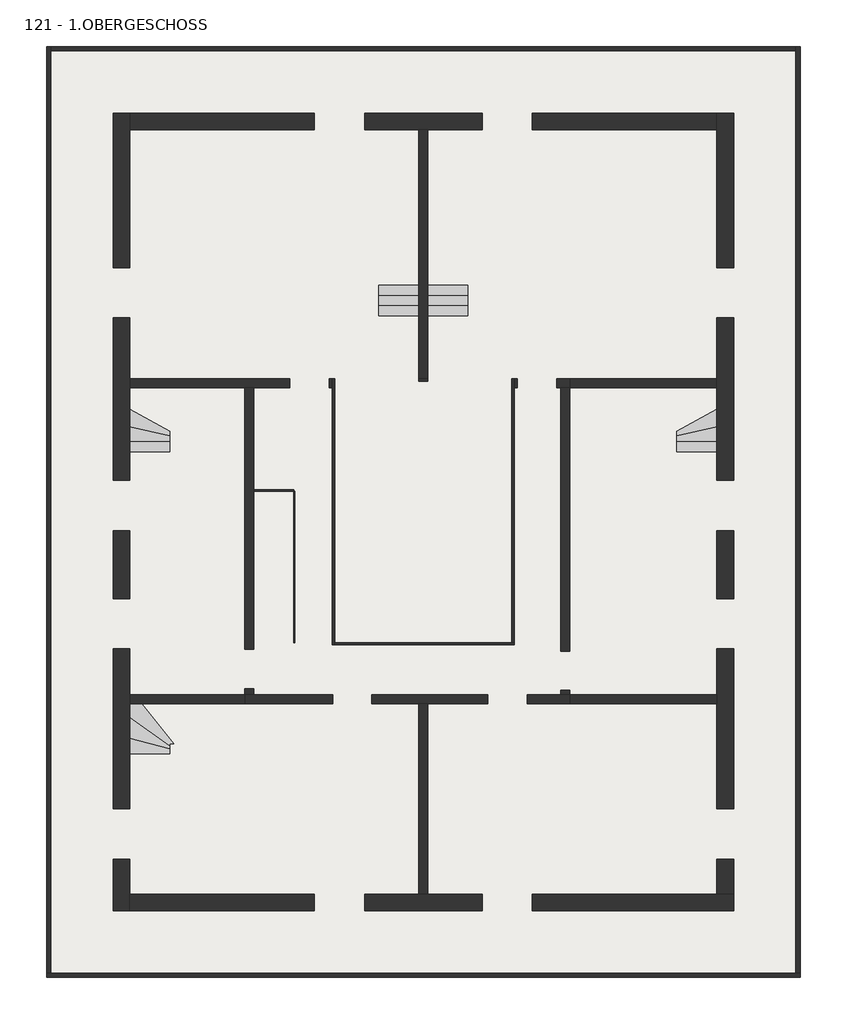
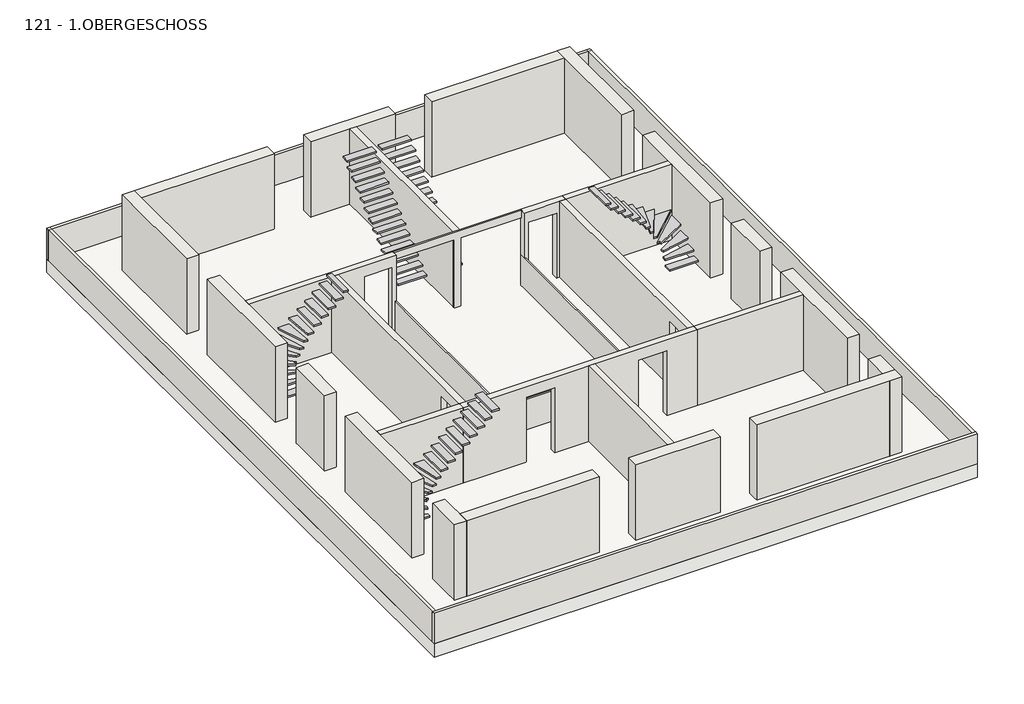
# One storey: 24 walls, 10 stairs, 1 slab.
"""IFC4 building model written with IfcOpenShell, lengths in millimetres."""

import ifcopenshell
import ifcopenshell.guid

model = None  # the IFC model being written
_history = None  # IfcOwnerHistory: only IFC2X3 demands one
_inside = {}  # id of a spatial element -> (the spatial element, [elements in it])
_under = {}  # id of a project, library or spatial element -> (it, [spatial elements below it])
_declared = {}  # id of a project -> (the project, [libraries it declares])
_typed = {}  # id of a type object -> (the type object, [elements of that type])
_made_of = {}  # id of a material, layer set ... -> (it, [elements and type objects made of it])


def new_model(schema):
    """Start an empty IFC model of exactly this schema.

    Asked for "IFC4X3", IfcOpenShell would pick the latest addendum, in which some entities
    have other attributes; the version numbers below select the first issue.
    IFC2X3 requires an IfcOwnerHistory on every rooted entity: one is made here for all.
    """
    global model, _history
    if schema == "IFC4X3":
        model = ifcopenshell.file(schema_version=(4, 3, 0, 0))
    else:
        model = ifcopenshell.file(schema=schema)
    _inside.clear()
    _under.clear()
    _declared.clear()
    _typed.clear()
    _made_of.clear()
    _history = None
    if model.schema == "IFC2X3":
        org = make("IfcOrganization", Name="unknown")
        user = make(
            "IfcPersonAndOrganization",
            ThePerson=make("IfcPerson", FamilyName="unknown"),
            TheOrganization=org,
        )
        app = make(
            "IfcApplication",
            ApplicationDeveloper=org,
            Version="unknown",
            ApplicationFullName="unknown",
            ApplicationIdentifier="unknown",
        )
        _history = make(
            "IfcOwnerHistory",
            OwningUser=user,
            OwningApplication=app,
            ChangeAction="ADDED",
            CreationDate=0,
        )
    return model


def make(cls, **values):
    """One entity of the class cls with the attributes given. An attribute that is None is left unset."""
    return model.create_entity(
        cls, **{name: value for name, value in values.items() if value is not None}
    )


def rooted(cls, **values):
    """An entity with a GlobalId (a new one), such as an element, a storey or a relation."""
    return make(cls, GlobalId=ifcopenshell.guid.new(), OwnerHistory=_history, **values)


def si_unit(unit_type, name, prefix=None):
    """IfcSIUnit, for example si_unit("LENGTHUNIT", "METRE", prefix="MILLI")."""
    return make("IfcSIUnit", UnitType=unit_type, Prefix=prefix, Name=name)


def assignment(units):
    """IfcUnitAssignment: the units of a project."""
    return None if units is None else make("IfcUnitAssignment", Units=units)


def point(xyz):
    """IfcCartesianPoint."""
    return None if xyz is None else make("IfcCartesianPoint", Coordinates=xyz)


def direction(xyz):
    """IfcDirection."""
    return None if xyz is None else make("IfcDirection", DirectionRatios=xyz)


def frame(location, z_axis=None, x_axis=None):
    """IfcAxis2Placement3D, a coordinate frame: its origin and axes. An axis left out is left unset."""
    return make(
        "IfcAxis2Placement3D",
        Location=point(location),
        Axis=direction(z_axis),
        RefDirection=direction(x_axis),
    )


def origin():
    """The frame at (0, 0, 0) with its axes left unset."""
    return frame((0.0, 0.0, 0.0))


def place(relative_to, where):
    """IfcLocalPlacement: puts the frame where relative to a parent placement (None: the world)."""
    return make(
        "IfcLocalPlacement", PlacementRelTo=relative_to, RelativePlacement=where
    )


def context(
    kind, dimensions, precision=None, world=None, true_north=None, identifier=None
):
    """IfcGeometricRepresentationContext, for example the 3D "Model" context."""
    return make(
        "IfcGeometricRepresentationContext",
        ContextIdentifier=identifier,
        ContextType=kind,
        CoordinateSpaceDimension=dimensions,
        Precision=precision,
        WorldCoordinateSystem=world,
        TrueNorth=true_north,
    )


def project(units=None, contexts=None):
    """IfcProject with its units and contexts."""
    return rooted(
        "IfcProject",
        Name="project",
        RepresentationContexts=contexts,
        UnitsInContext=assignment(units),
    )


def spatial(cls, under=None, at=None, **own):
    """A site, building, storey or space (cls), placed at a placement, below another one or the project."""
    s = rooted(cls, ObjectPlacement=at, **own)
    if under is not None:
        _under.setdefault(under.id(), (under, []))[1].append(s)
    return s


def polyline(points):
    """IfcPolyline through the points."""
    return make("IfcPolyline", Points=[point(p) for p in points])


def outline(outer, holes=None, kind="AREA"):
    """IfcArbitraryClosedProfileDef: a profile drawn as a closed curve; with holes, ...WithVoids."""
    if holes is None:
        return make("IfcArbitraryClosedProfileDef", ProfileType=kind, OuterCurve=outer)
    return make(
        "IfcArbitraryProfileDefWithVoids",
        ProfileType=kind,
        OuterCurve=outer,
        InnerCurves=holes,
    )


def extrude(swept, where, along, depth):
    """IfcExtrudedAreaSolid: the profile swept, set in the frame where, extruded along a direction by depth."""
    return make(
        "IfcExtrudedAreaSolid",
        SweptArea=swept,
        Position=where,
        ExtrudedDirection=direction(along),
        Depth=depth,
    )


def shape(context_of_items, identifier, shape_type, items):
    """IfcShapeRepresentation: the items that make up one representation, for example the "Body"."""
    return make(
        "IfcShapeRepresentation",
        ContextOfItems=context_of_items,
        RepresentationIdentifier=identifier,
        RepresentationType=shape_type,
        Items=items,
    )


def source(mapping_origin, context_of_items, identifier, shape_type, items):
    """IfcRepresentationMap: a shape defined once, which mapped items show again and again."""
    return make(
        "IfcRepresentationMap",
        MappingOrigin=mapping_origin,
        MappedRepresentation=shape(context_of_items, identifier, shape_type, items),
    )


def transform(
    local_origin,
    x_axis=None,
    y_axis=None,
    z_axis=None,
    scale=None,
    scale2=None,
    scale3=None,
    uniform=True,
):
    """IfcCartesianTransformationOperator3D, or its non-uniform kind. x_axis, y_axis, z_axis: its Axis1, 2, 3."""
    if uniform:
        return make(
            "IfcCartesianTransformationOperator3D",
            Axis1=direction(x_axis),
            Axis2=direction(y_axis),
            LocalOrigin=point(local_origin),
            Scale=scale,
            Axis3=direction(z_axis),
        )
    return make(
        "IfcCartesianTransformationOperator3DnonUniform",
        Axis1=direction(x_axis),
        Axis2=direction(y_axis),
        LocalOrigin=point(local_origin),
        Scale=scale,
        Axis3=direction(z_axis),
        Scale2=scale2,
        Scale3=scale3,
    )


def mapped(mapping_source, mapping_target):
    """IfcMappedItem: shows the shape of a source again, moved by a transform."""
    return make(
        "IfcMappedItem", MappingSource=mapping_source, MappingTarget=mapping_target
    )


def made_of(thing, what):
    """Note that an element or type object is made of a material, layer set ...; save() writes the relation."""
    if what is not None:
        _made_of.setdefault(what.id(), (what, []))[1].append(thing)
    return thing


def element(
    cls,
    number,
    at=None,
    inside=None,
    cuts=None,
    type_object=None,
    material=None,
    context=None,
    identifier="Body",
    shape_type=None,
    held_by="IfcProductDefinitionShape",
    body=None,
    shapes=None,
    **own,
):
    """One element of the class cls, such as IfcWall. Its Tag is "e" and its number.

    at: its placement. inside: the storey or other place that contains it. cuts: it is an
    opening in that element (IfcRelVoidsElement). A single representation is given by context,
    identifier, shape_type and body (its items); several are given by shapes. held_by: the class
    of the entity that holds the representations. save() writes the other relations.
    """
    e = rooted(cls, Tag="e%d" % number, ObjectPlacement=at, **own)
    if body is not None:
        shapes = [shape(context, identifier, shape_type, body)]
    if shapes is not None:
        e.Representation = make(held_by, Representations=shapes)
    if inside is not None:
        _inside.setdefault(inside.id(), (inside, []))[1].append(e)
    if cuts is not None:
        rooted(
            "IfcRelVoidsElement", RelatingBuildingElement=cuts, RelatedOpeningElement=e
        )
    if type_object is not None:
        _typed.setdefault(type_object.id(), (type_object, []))[1].append(e)
    return made_of(e, material)


def aggregate(whole, parts):
    """IfcRelAggregates: a whole, such as a stair, and the parts it consists of."""
    return rooted("IfcRelAggregates", RelatingObject=whole, RelatedObjects=parts)


def save(model, path):
    """Write the relations noted so far, then the file.

    IfcRelAggregates (storeys below a building ...), IfcRelContainedInSpatialStructure (elements
    in a storey), IfcRelDefinesByType, IfcRelAssociatesMaterial and IfcRelDeclares: one each for
    every whole, place, type object, material and project.
    """
    for whole, parts in _under.values():
        aggregate(whole, parts)
    for where, things in _inside.values():
        rooted(
            "IfcRelContainedInSpatialStructure",
            RelatedElements=things,
            RelatingStructure=where,
        )
    for kind, things in _typed.values():
        rooted("IfcRelDefinesByType", RelatedObjects=things, RelatingType=kind)
    for what, things in _made_of.values():
        rooted("IfcRelAssociatesMaterial", RelatedObjects=things, RelatingMaterial=what)
    for by, libraries in _declared.values():
        rooted("IfcRelDeclares", RelatingContext=by, RelatedDefinitions=libraries)
    model.write(path)


def slab_4f2d1623(model_context):
    return source(origin(), model_context, "Body", "SweptSolid", [
        extrude(outline(polyline([(174297.7593015, 47984.7962965), (174297.7593015, 26981.9343946), (157297.7593015, 26981.9343946), (157297.7593015, 47984.7962965), (174297.7593015, 47984.7962965)])), frame((0.0, 0.0, 2880.0), z_axis=(0.0, 0.0, 1.0), x_axis=(1.0, 0.0, 0.0)), (0.0, 0.0, 1.0), 450.0),
    ])


def stair_92ba3d55(model_context):
    return source(origin(), model_context, "Body", "SweptSolid", [
        extrude(outline(polyline([(160077.7593015, 32139.1812131), (160077.7593015, 32029.7962965), (159177.7593015, 32029.7962965), (159177.7593015, 32381.5903923), (160077.7593015, 32139.1812131)])), frame((0.0, 0.0, 3480.0), z_axis=(0.0, 0.0, 1.0), x_axis=(1.0, 0.0, 0.0)), (0.0, 0.0, 1.0), 50.0),
        extrude(outline(polyline([(160077.7593015, 32208.6851854), (160077.7593015, 32139.1812131), (159177.7593015, 32381.5903923), (159177.7593015, 32851.1265298), (160077.7593015, 32208.6851854)])), frame((0.0, 0.0, 3680.0), z_axis=(0.0, 0.0, 1.0), x_axis=(1.0, 0.0, 0.0)), (0.0, 0.0, 1.0), 50.0),
        extrude(outline(polyline([(159450.38828, 33159.7962965), (160164.4298971, 32259.7962965), (160077.7593015, 32259.7962965), (160077.7593015, 32208.6851854), (159177.7593015, 32851.1265298), (159177.7593015, 33159.7962965), (159450.38828, 33159.7962965)])), frame((0.0, 0.0, 3880.0), z_axis=(0.0, 0.0, 1.0), x_axis=(1.0, 0.0, 0.0)), (0.0, 0.0, 1.0), 50.0),
        extrude(outline(polyline([(160285.4396784, 32259.7962965), (160164.4298971, 32259.7962965), (159450.38828, 33159.7962965), (159877.5404106, 33159.7962965), (160285.4396784, 32259.7962965)])), frame((0.0, 0.0, 4080.0), z_axis=(0.0, 0.0, 1.0), x_axis=(1.0, 0.0, 0.0)), (0.0, 0.0, 1.0), 50.0),
        extrude(outline(polyline([(160412.2916695, 32259.7962965), (160285.4396784, 32259.7962965), (159877.5404106, 33159.7962965), (160212.4306066, 33159.7962965), (160412.2916695, 32259.7962965)])), frame((0.0, 0.0, 4280.0), z_axis=(0.0, 0.0, 1.0), x_axis=(1.0, 0.0, 0.0)), (0.0, 0.0, 1.0), 50.0),
        extrude(outline(polyline([(160546.5910216, 32259.7962965), (160412.2916695, 32259.7962965), (160212.4306066, 33159.7962965), (160538.1312545, 33159.7962965), (160546.5910216, 32259.7962965)])), frame((0.0, 0.0, 4480.0), z_axis=(0.0, 0.0, 1.0), x_axis=(1.0, 0.0, 0.0)), (0.0, 0.0, 1.0), 50.0),
        extrude(outline(polyline([(160772.3611381, 32259.7962965), (160546.5910216, 32259.7962965), (160538.1312545, 33159.7962965), (160772.3611381, 33159.7962965), (160772.3611381, 32259.7962965)])), frame((0.0, 0.0, 4680.0), z_axis=(0.0, 0.0, 1.0), x_axis=(1.0, 0.0, 0.0)), (0.0, 0.0, 1.0), 50.0),
        extrude(outline(polyline([(161002.3611381, 32259.7962965), (160772.3611381, 32259.7962965), (160772.3611381, 33159.7962965), (161002.3611381, 33159.7962965), (161002.3611381, 32259.7962965)])), frame((0.0, 0.0, 4880.0), z_axis=(0.0, 0.0, 1.0), x_axis=(1.0, 0.0, 0.0)), (0.0, 0.0, 1.0), 50.0),
        extrude(outline(polyline([(161232.3611381, 32259.7962965), (161002.3611381, 32259.7962965), (161002.3611381, 33159.7962965), (161232.3611381, 33159.7962965), (161232.3611381, 32259.7962965)])), frame((0.0, 0.0, 5080.0), z_axis=(0.0, 0.0, 1.0), x_axis=(1.0, 0.0, 0.0)), (0.0, 0.0, 1.0), 50.0),
        extrude(outline(polyline([(161462.3611381, 32259.7962965), (161232.3611381, 32259.7962965), (161232.3611381, 33159.7962965), (161462.3611381, 33159.7962965), (161462.3611381, 32259.7962965)])), frame((0.0, 0.0, 5280.0), z_axis=(0.0, 0.0, 1.0), x_axis=(1.0, 0.0, 0.0)), (0.0, 0.0, 1.0), 50.0),
        extrude(outline(polyline([(161692.3611381, 32259.7962965), (161462.3611381, 32259.7962965), (161462.3611381, 33159.7962965), (161692.3611381, 33159.7962965), (161692.3611381, 32259.7962965)])), frame((0.0, 0.0, 5480.0), z_axis=(0.0, 0.0, 1.0), x_axis=(1.0, 0.0, 0.0)), (0.0, 0.0, 1.0), 50.0),
        extrude(outline(polyline([(161922.3611381, 32259.7962965), (161692.3611381, 32259.7962965), (161692.3611381, 33159.7962965), (161922.3611381, 33159.7962965), (161922.3611381, 32259.7962965)])), frame((0.0, 0.0, 5680.0), z_axis=(0.0, 0.0, 1.0), x_axis=(1.0, 0.0, 0.0)), (0.0, 0.0, 1.0), 50.0),
        extrude(outline(polyline([(162152.3611381, 32259.7962965), (161922.3611381, 32259.7962965), (161922.3611381, 33159.7962965), (162152.3611381, 33159.7962965), (162152.3611381, 32259.7962965)])), frame((0.0, 0.0, 5880.0), z_axis=(0.0, 0.0, 1.0), x_axis=(1.0, 0.0, 0.0)), (0.0, 0.0, 1.0), 50.0),
        extrude(outline(polyline([(162382.3611381, 32259.7962965), (162152.3611381, 32259.7962965), (162152.3611381, 33159.7962965), (162382.3611381, 33159.7962965), (162382.3611381, 32259.7962965)])), frame((0.0, 0.0, 6080.0), z_axis=(0.0, 0.0, 1.0), x_axis=(1.0, 0.0, 0.0)), (0.0, 0.0, 1.0), 50.0),
    ])


def stair_5d17669e(model_context):
    return source(origin(), model_context, "Body", "SweptSolid", [
        extrude(outline(polyline([(166797.7593015, 42144.7962965), (166797.7593015, 41914.7962965), (165897.7593015, 41914.7962965), (165897.7593015, 42144.7962965), (166797.7593015, 42144.7962965)])), frame((0.0, 0.0, 3482.1428571), z_axis=(0.0, 0.0, 1.0), x_axis=(1.0, 0.0, 0.0)), (0.0, 0.0, 1.0), 50.0),
        extrude(outline(polyline([(166797.7593015, 42374.7962965), (166797.7593015, 42144.7962965), (165897.7593015, 42144.7962965), (165897.7593015, 42374.7962965), (166797.7593015, 42374.7962965)])), frame((0.0, 0.0, 3684.2857143), z_axis=(0.0, 0.0, 1.0), x_axis=(1.0, 0.0, 0.0)), (0.0, 0.0, 1.0), 50.0),
        extrude(outline(polyline([(166797.7593015, 42604.7962965), (166797.7593015, 42374.7962965), (165897.7593015, 42374.7962965), (165897.7593015, 42604.7962965), (166797.7593015, 42604.7962965)])), frame((0.0, 0.0, 3886.4285714), z_axis=(0.0, 0.0, 1.0), x_axis=(1.0, 0.0, 0.0)), (0.0, 0.0, 1.0), 50.0),
        extrude(outline(polyline([(166797.7593015, 42834.7962965), (166797.7593015, 42604.7962965), (165897.7593015, 42604.7962965), (165897.7593015, 42834.7962965), (166797.7593015, 42834.7962965)])), frame((0.0, 0.0, 4088.5714286), z_axis=(0.0, 0.0, 1.0), x_axis=(1.0, 0.0, 0.0)), (0.0, 0.0, 1.0), 50.0),
        extrude(outline(polyline([(166797.7593015, 43064.7962965), (166797.7593015, 42834.7962965), (165897.7593015, 42834.7962965), (165897.7593015, 43064.7962965), (166797.7593015, 43064.7962965)])), frame((0.0, 0.0, 4290.7142857), z_axis=(0.0, 0.0, 1.0), x_axis=(1.0, 0.0, 0.0)), (0.0, 0.0, 1.0), 50.0),
        extrude(outline(polyline([(166797.7593015, 43294.7962965), (166797.7593015, 43064.7962965), (165897.7593015, 43064.7962965), (165897.7593015, 43294.7962965), (166797.7593015, 43294.7962965)])), frame((0.0, 0.0, 4492.8571429), z_axis=(0.0, 0.0, 1.0), x_axis=(1.0, 0.0, 0.0)), (0.0, 0.0, 1.0), 50.0),
        extrude(outline(polyline([(166797.7593015, 43524.7962965), (166797.7593015, 43294.7962965), (165897.7593015, 43294.7962965), (165897.7593015, 43524.7962965), (166797.7593015, 43524.7962965)])), frame((0.0, 0.0, 4695.0), z_axis=(0.0, 0.0, 1.0), x_axis=(1.0, 0.0, 0.0)), (0.0, 0.0, 1.0), 50.0),
        extrude(outline(polyline([(166797.7593015, 43754.7962965), (166797.7593015, 43524.7962965), (165897.7593015, 43524.7962965), (165897.7593015, 43754.7962965), (166797.7593015, 43754.7962965)])), frame((0.0, 0.0, 4897.1428571), z_axis=(0.0, 0.0, 1.0), x_axis=(1.0, 0.0, 0.0)), (0.0, 0.0, 1.0), 50.0),
        extrude(outline(polyline([(166797.7593015, 43984.7962965), (166797.7593015, 43754.7962965), (165897.7593015, 43754.7962965), (165897.7593015, 43984.7962965), (166797.7593015, 43984.7962965)])), frame((0.0, 0.0, 5099.2857143), z_axis=(0.0, 0.0, 1.0), x_axis=(1.0, 0.0, 0.0)), (0.0, 0.0, 1.0), 50.0),
        extrude(outline(polyline([(166797.7593015, 44214.7962965), (166797.7593015, 43984.7962965), (165897.7593015, 43984.7962965), (165897.7593015, 44214.7962965), (166797.7593015, 44214.7962965)])), frame((0.0, 0.0, 5301.4285714), z_axis=(0.0, 0.0, 1.0), x_axis=(1.0, 0.0, 0.0)), (0.0, 0.0, 1.0), 50.0),
        extrude(outline(polyline([(166797.7593015, 44444.7962965), (166797.7593015, 44214.7962965), (165897.7593015, 44214.7962965), (165897.7593015, 44444.7962965), (166797.7593015, 44444.7962965)])), frame((0.0, 0.0, 5503.5714286), z_axis=(0.0, 0.0, 1.0), x_axis=(1.0, 0.0, 0.0)), (0.0, 0.0, 1.0), 50.0),
        extrude(outline(polyline([(166797.7593015, 44674.7962965), (166797.7593015, 44444.7962965), (165897.7593015, 44444.7962965), (165897.7593015, 44674.7962965), (166797.7593015, 44674.7962965)])), frame((0.0, 0.0, 5705.7142857), z_axis=(0.0, 0.0, 1.0), x_axis=(1.0, 0.0, 0.0)), (0.0, 0.0, 1.0), 50.0),
        extrude(outline(polyline([(166797.7593015, 44904.7962965), (166797.7593015, 44674.7962965), (165897.7593015, 44674.7962965), (165897.7593015, 44904.7962965), (166797.7593015, 44904.7962965)])), frame((0.0, 0.0, 5907.8571429), z_axis=(0.0, 0.0, 1.0), x_axis=(1.0, 0.0, 0.0)), (0.0, 0.0, 1.0), 50.0),
    ])


def stair_42ef58a3(model_context):
    return source(origin(), model_context, "Body", "SweptSolid", [
        extrude(outline(polyline([(165697.7593015, 42144.7962965), (165697.7593015, 41914.7962965), (164797.7593015, 41914.7962965), (164797.7593015, 42144.7962965), (165697.7593015, 42144.7962965)])), frame((0.0, 0.0, 3482.1428571), z_axis=(0.0, 0.0, 1.0), x_axis=(1.0, 0.0, 0.0)), (0.0, 0.0, 1.0), 50.0),
        extrude(outline(polyline([(165697.7593015, 42374.7962965), (165697.7593015, 42144.7962965), (164797.7593015, 42144.7962965), (164797.7593015, 42374.7962965), (165697.7593015, 42374.7962965)])), frame((0.0, 0.0, 3684.2857143), z_axis=(0.0, 0.0, 1.0), x_axis=(1.0, 0.0, 0.0)), (0.0, 0.0, 1.0), 50.0),
        extrude(outline(polyline([(165697.7593015, 42604.7962965), (165697.7593015, 42374.7962965), (164797.7593015, 42374.7962965), (164797.7593015, 42604.7962965), (165697.7593015, 42604.7962965)])), frame((0.0, 0.0, 3886.4285714), z_axis=(0.0, 0.0, 1.0), x_axis=(1.0, 0.0, 0.0)), (0.0, 0.0, 1.0), 50.0),
        extrude(outline(polyline([(165697.7593015, 42834.7962965), (165697.7593015, 42604.7962965), (164797.7593015, 42604.7962965), (164797.7593015, 42834.7962965), (165697.7593015, 42834.7962965)])), frame((0.0, 0.0, 4088.5714286), z_axis=(0.0, 0.0, 1.0), x_axis=(1.0, 0.0, 0.0)), (0.0, 0.0, 1.0), 50.0),
        extrude(outline(polyline([(165697.7593015, 43064.7962965), (165697.7593015, 42834.7962965), (164797.7593015, 42834.7962965), (164797.7593015, 43064.7962965), (165697.7593015, 43064.7962965)])), frame((0.0, 0.0, 4290.7142857), z_axis=(0.0, 0.0, 1.0), x_axis=(1.0, 0.0, 0.0)), (0.0, 0.0, 1.0), 50.0),
        extrude(outline(polyline([(165697.7593015, 43294.7962965), (165697.7593015, 43064.7962965), (164797.7593015, 43064.7962965), (164797.7593015, 43294.7962965), (165697.7593015, 43294.7962965)])), frame((0.0, 0.0, 4492.8571429), z_axis=(0.0, 0.0, 1.0), x_axis=(1.0, 0.0, 0.0)), (0.0, 0.0, 1.0), 50.0),
        extrude(outline(polyline([(165697.7593015, 43524.7962965), (165697.7593015, 43294.7962965), (164797.7593015, 43294.7962965), (164797.7593015, 43524.7962965), (165697.7593015, 43524.7962965)])), frame((0.0, 0.0, 4695.0), z_axis=(0.0, 0.0, 1.0), x_axis=(1.0, 0.0, 0.0)), (0.0, 0.0, 1.0), 50.0),
        extrude(outline(polyline([(165697.7593015, 43754.7962965), (165697.7593015, 43524.7962965), (164797.7593015, 43524.7962965), (164797.7593015, 43754.7962965), (165697.7593015, 43754.7962965)])), frame((0.0, 0.0, 4897.1428571), z_axis=(0.0, 0.0, 1.0), x_axis=(1.0, 0.0, 0.0)), (0.0, 0.0, 1.0), 50.0),
        extrude(outline(polyline([(165697.7593015, 43984.7962965), (165697.7593015, 43754.7962965), (164797.7593015, 43754.7962965), (164797.7593015, 43984.7962965), (165697.7593015, 43984.7962965)])), frame((0.0, 0.0, 5099.2857143), z_axis=(0.0, 0.0, 1.0), x_axis=(1.0, 0.0, 0.0)), (0.0, 0.0, 1.0), 50.0),
        extrude(outline(polyline([(165697.7593015, 44214.7962965), (165697.7593015, 43984.7962965), (164797.7593015, 43984.7962965), (164797.7593015, 44214.7962965), (165697.7593015, 44214.7962965)])), frame((0.0, 0.0, 5301.4285714), z_axis=(0.0, 0.0, 1.0), x_axis=(1.0, 0.0, 0.0)), (0.0, 0.0, 1.0), 50.0),
        extrude(outline(polyline([(165697.7593015, 44444.7962965), (165697.7593015, 44214.7962965), (164797.7593015, 44214.7962965), (164797.7593015, 44444.7962965), (165697.7593015, 44444.7962965)])), frame((0.0, 0.0, 5503.5714286), z_axis=(0.0, 0.0, 1.0), x_axis=(1.0, 0.0, 0.0)), (0.0, 0.0, 1.0), 50.0),
        extrude(outline(polyline([(165697.7593015, 44674.7962965), (165697.7593015, 44444.7962965), (164797.7593015, 44444.7962965), (164797.7593015, 44674.7962965), (165697.7593015, 44674.7962965)])), frame((0.0, 0.0, 5705.7142857), z_axis=(0.0, 0.0, 1.0), x_axis=(1.0, 0.0, 0.0)), (0.0, 0.0, 1.0), 50.0),
        extrude(outline(polyline([(165697.7593015, 44904.7962965), (165697.7593015, 44674.7962965), (164797.7593015, 44674.7962965), (164797.7593015, 44904.7962965), (165697.7593015, 44904.7962965)])), frame((0.0, 0.0, 5907.8571429), z_axis=(0.0, 0.0, 1.0), x_axis=(1.0, 0.0, 0.0)), (0.0, 0.0, 1.0), 50.0),
    ])


def stair_4856ba97(model_context):
    return source(origin(), model_context, "Body", "SweptSolid", [
        extrude(outline(polyline([(159177.7593015, 39074.7962965), (160077.7593015, 39074.7962965), (160077.7593015, 38844.7962965), (159177.7593015, 38844.7962965), (159177.7593015, 39074.7962965)])), frame((0.0, 0.0, 3482.1428571), z_axis=(0.0, 0.0, 1.0), x_axis=(1.0, 0.0, 0.0)), (0.0, 0.0, 1.0), 50.0),
        extrude(outline(polyline([(159177.7593015, 39407.7634868), (160077.7593015, 39201.8291061), (160077.7593015, 39074.7962965), (159177.7593015, 39074.7962965), (159177.7593015, 39407.7634868)])), frame((0.0, 0.0, 3684.2857143), z_axis=(0.0, 0.0, 1.0), x_axis=(1.0, 0.0, 0.0)), (0.0, 0.0, 1.0), 50.0),
        extrude(outline(polyline([(159177.7593015, 39801.0914939), (160077.7593015, 39301.7193734), (160077.7593015, 39201.8291061), (159177.7593015, 39407.7634868), (159177.7593015, 39801.0914939)])), frame((0.0, 0.0, 3886.4285714), z_axis=(0.0, 0.0, 1.0), x_axis=(1.0, 0.0, 0.0)), (0.0, 0.0, 1.0), 50.0),
        extrude(outline(polyline([(159177.7593015, 40284.7962965), (159200.4297176, 40284.7962965), (160147.7593015, 39384.7962965), (160077.7593015, 39384.7962965), (160077.7593015, 39301.7193734), (159177.7593015, 39801.0914939), (159177.7593015, 40284.7962965)])), frame((0.0, 0.0, 4088.5714286), z_axis=(0.0, 0.0, 1.0), x_axis=(1.0, 0.0, 0.0)), (0.0, 0.0, 1.0), 50.0),
        extrude(outline(polyline([(159730.1980238, 40284.7962965), (160258.7713888, 39384.7962965), (160147.7593015, 39384.7962965), (159200.4297176, 40284.7962965), (159730.1980238, 40284.7962965)])), frame((0.0, 0.0, 4290.7142857), z_axis=(0.0, 0.0, 1.0), x_axis=(1.0, 0.0, 0.0)), (0.0, 0.0, 1.0), 50.0),
        extrude(outline(polyline([(160089.4284981, 40284.7962965), (160375.293778, 39384.7962965), (160258.7713888, 39384.7962965), (159730.1980238, 40284.7962965), (160089.4284981, 40284.7962965)])), frame((0.0, 0.0, 4492.8571429), z_axis=(0.0, 0.0, 1.0), x_axis=(1.0, 0.0, 0.0)), (0.0, 0.0, 1.0), 50.0),
        extrude(outline(polyline([(160425.6183342, 40284.7962965), (160499.1039419, 39384.7962965), (160375.293778, 39384.7962965), (160089.4284981, 40284.7962965), (160425.6183342, 40284.7962965)])), frame((0.0, 0.0, 4695.0), z_axis=(0.0, 0.0, 1.0), x_axis=(1.0, 0.0, 0.0)), (0.0, 0.0, 1.0), 50.0),
        extrude(outline(polyline([(160692.3611381, 40284.7962965), (160692.3611381, 39384.7962965), (160499.1039419, 39384.7962965), (160425.6183342, 40284.7962965), (160692.3611381, 40284.7962965)])), frame((0.0, 0.0, 4897.1428571), z_axis=(0.0, 0.0, 1.0), x_axis=(1.0, 0.0, 0.0)), (0.0, 0.0, 1.0), 50.0),
        extrude(outline(polyline([(160922.3611381, 40284.7962965), (160922.3611381, 39384.7962965), (160692.3611381, 39384.7962965), (160692.3611381, 40284.7962965), (160922.3611381, 40284.7962965)])), frame((0.0, 0.0, 5099.2857143), z_axis=(0.0, 0.0, 1.0), x_axis=(1.0, 0.0, 0.0)), (0.0, 0.0, 1.0), 50.0),
        extrude(outline(polyline([(161152.3611381, 40284.7962965), (161152.3611381, 39384.7962965), (160922.3611381, 39384.7962965), (160922.3611381, 40284.7962965), (161152.3611381, 40284.7962965)])), frame((0.0, 0.0, 5301.4285714), z_axis=(0.0, 0.0, 1.0), x_axis=(1.0, 0.0, 0.0)), (0.0, 0.0, 1.0), 50.0),
        extrude(outline(polyline([(161382.3611381, 40284.7962965), (161382.3611381, 39384.7962965), (161152.3611381, 39384.7962965), (161152.3611381, 40284.7962965), (161382.3611381, 40284.7962965)])), frame((0.0, 0.0, 5503.5714286), z_axis=(0.0, 0.0, 1.0), x_axis=(1.0, 0.0, 0.0)), (0.0, 0.0, 1.0), 50.0),
        extrude(outline(polyline([(161612.3611381, 40284.7962965), (161612.3611381, 39384.7962965), (161382.3611381, 39384.7962965), (161382.3611381, 40284.7962965), (161612.3611381, 40284.7962965)])), frame((0.0, 0.0, 5705.7142857), z_axis=(0.0, 0.0, 1.0), x_axis=(1.0, 0.0, 0.0)), (0.0, 0.0, 1.0), 50.0),
        extrude(outline(polyline([(161772.7593015, 40284.7962965), (161772.7593015, 39384.7962965), (161612.3611381, 39384.7962965), (161612.3611381, 40284.7962965), (161772.7593015, 40284.7962965)])), frame((0.0, 0.0, 5907.8571429), z_axis=(0.0, 0.0, 1.0), x_axis=(1.0, 0.0, 0.0)), (0.0, 0.0, 1.0), 50.0),
    ])


def stair_6893023c(model_context):
    return source(origin(), model_context, "Body", "SweptSolid", [
        extrude(outline(polyline([(171517.7593015, 39074.7962965), (172417.7593015, 39074.7962965), (172417.7593015, 38844.7962965), (171517.7593015, 38844.7962965), (171517.7593015, 39074.7962965)])), frame((0.0, 0.0, 3482.1428571), z_axis=(0.0, 0.0, 1.0), x_axis=(1.0, 0.0, 0.0)), (0.0, 0.0, 1.0), 50.0),
        extrude(outline(polyline([(171517.7593015, 39201.8291061), (172417.7593015, 39407.7634868), (172417.7593015, 39074.7962965), (171517.7593015, 39074.7962965), (171517.7593015, 39201.8291061)])), frame((0.0, 0.0, 3684.2857143), z_axis=(0.0, 0.0, 1.0), x_axis=(1.0, 0.0, 0.0)), (0.0, 0.0, 1.0), 50.0),
        extrude(outline(polyline([(171517.7593015, 39301.7193734), (172417.7593015, 39801.0914939), (172417.7593015, 39407.7634868), (171517.7593015, 39201.8291061), (171517.7593015, 39301.7193734)])), frame((0.0, 0.0, 3886.4285714), z_axis=(0.0, 0.0, 1.0), x_axis=(1.0, 0.0, 0.0)), (0.0, 0.0, 1.0), 50.0),
        extrude(outline(polyline([(171517.7593015, 39384.7962965), (171447.7593015, 39384.7962965), (172395.0888853, 40284.7962965), (172417.7593015, 40284.7962965), (172417.7593015, 39801.0914939), (171517.7593015, 39301.7193734), (171517.7593015, 39384.7962965)])), frame((0.0, 0.0, 4088.5714286), z_axis=(0.0, 0.0, 1.0), x_axis=(1.0, 0.0, 0.0)), (0.0, 0.0, 1.0), 50.0),
        extrude(outline(polyline([(171336.7472141, 39384.7962965), (171865.3205791, 40284.7962965), (172395.0888853, 40284.7962965), (171447.7593015, 39384.7962965), (171336.7472141, 39384.7962965)])), frame((0.0, 0.0, 4290.7142857), z_axis=(0.0, 0.0, 1.0), x_axis=(1.0, 0.0, 0.0)), (0.0, 0.0, 1.0), 50.0),
        extrude(outline(polyline([(171220.2248249, 39384.7962965), (171506.0901048, 40284.7962965), (171865.3205791, 40284.7962965), (171336.7472141, 39384.7962965), (171220.2248249, 39384.7962965)])), frame((0.0, 0.0, 4492.8571429), z_axis=(0.0, 0.0, 1.0), x_axis=(1.0, 0.0, 0.0)), (0.0, 0.0, 1.0), 50.0),
        extrude(outline(polyline([(171096.414661, 39384.7962965), (171169.9002687, 40284.7962965), (171506.0901048, 40284.7962965), (171220.2248249, 39384.7962965), (171096.414661, 39384.7962965)])), frame((0.0, 0.0, 4695.0), z_axis=(0.0, 0.0, 1.0), x_axis=(1.0, 0.0, 0.0)), (0.0, 0.0, 1.0), 50.0),
        extrude(outline(polyline([(170903.1574649, 39384.7962965), (170903.1574649, 40284.7962965), (171169.9002687, 40284.7962965), (171096.414661, 39384.7962965), (170903.1574649, 39384.7962965)])), frame((0.0, 0.0, 4897.1428571), z_axis=(0.0, 0.0, 1.0), x_axis=(1.0, 0.0, 0.0)), (0.0, 0.0, 1.0), 50.0),
        extrude(outline(polyline([(170673.1574649, 39384.7962965), (170673.1574649, 40284.7962965), (170903.1574649, 40284.7962965), (170903.1574649, 39384.7962965), (170673.1574649, 39384.7962965)])), frame((0.0, 0.0, 5099.2857143), z_axis=(0.0, 0.0, 1.0), x_axis=(1.0, 0.0, 0.0)), (0.0, 0.0, 1.0), 50.0),
        extrude(outline(polyline([(170443.1574649, 39384.7962965), (170443.1574649, 40284.7962965), (170673.1574649, 40284.7962965), (170673.1574649, 39384.7962965), (170443.1574649, 39384.7962965)])), frame((0.0, 0.0, 5301.4285714), z_axis=(0.0, 0.0, 1.0), x_axis=(1.0, 0.0, 0.0)), (0.0, 0.0, 1.0), 50.0),
        extrude(outline(polyline([(170213.1574649, 39384.7962965), (170213.1574649, 40284.7962965), (170443.1574649, 40284.7962965), (170443.1574649, 39384.7962965), (170213.1574649, 39384.7962965)])), frame((0.0, 0.0, 5503.5714286), z_axis=(0.0, 0.0, 1.0), x_axis=(1.0, 0.0, 0.0)), (0.0, 0.0, 1.0), 50.0),
        extrude(outline(polyline([(169983.1574649, 39384.7962965), (169983.1574649, 40284.7962965), (170213.1574649, 40284.7962965), (170213.1574649, 39384.7962965), (169983.1574649, 39384.7962965)])), frame((0.0, 0.0, 5705.7142857), z_axis=(0.0, 0.0, 1.0), x_axis=(1.0, 0.0, 0.0)), (0.0, 0.0, 1.0), 50.0),
        extrude(outline(polyline([(169822.7593015, 39384.7962965), (169822.7593015, 40284.7962965), (169983.1574649, 40284.7962965), (169983.1574649, 39384.7962965), (169822.7593015, 39384.7962965)])), frame((0.0, 0.0, 5907.8571429), z_axis=(0.0, 0.0, 1.0), x_axis=(1.0, 0.0, 0.0)), (0.0, 0.0, 1.0), 50.0),
    ])


model = new_model("IFC4")

# Units and contexts
model_context = context("Model", 3, world=origin())
ifc_project = project(units=[si_unit("LENGTHUNIT", "METRE", prefix="MILLI")], contexts=[model_context])

# Site, building, storey
site = spatial("IfcSite", under=ifc_project)
building = spatial("IfcBuilding", under=site)
storey = spatial("IfcBuildingStorey", under=building, Name="121 - 1.OBERGESCHOSS", Elevation=2825.0)

# Slab
placement = place(None, origin())
slab_shape = slab_4f2d1623(model_context)
element("IfcSlab", 1, ObjectType="Holzdecke 176 : Holzdecke 176", at=placement, inside=storey, context=model_context, shape_type="MappedRepresentation", body=[
    mapped(slab_shape, transform((0.0, 0.0, 0.0), x_axis=(1.0, 0.0, 0.0), y_axis=(0.0, 1.0, 0.0), z_axis=(0.0, 0.0, 1.0))),
])

# Stairs
stair_shape = stair_92ba3d55(model_context)
element("IfcStair", 2, ObjectType="  97010 :   97010", at=placement, inside=storey, context=model_context, shape_type="MappedRepresentation", body=[
    mapped(stair_shape, transform((0.0, 0.0, 0.0), x_axis=(1.0, 0.0, 0.0), y_axis=(0.0, 1.0, 0.0), z_axis=(0.0, 0.0, 1.0))),
])
stair_2_shape = stair_5d17669e(model_context)
element("IfcStair", 3, ObjectType="  97882 :   97882", at=placement, inside=storey, context=model_context, shape_type="MappedRepresentation", body=[
    mapped(stair_2_shape, transform((0.0, 0.0, 0.0), x_axis=(1.0, 0.0, 0.0), y_axis=(0.0, 1.0, 0.0), z_axis=(0.0, 0.0, 1.0))),
])
stair_3_shape = stair_42ef58a3(model_context)
element("IfcStair", 4, ObjectType="  98300 :   98300", at=placement, inside=storey, context=model_context, shape_type="MappedRepresentation", body=[
    mapped(stair_3_shape, transform((0.0, 0.0, 0.0), x_axis=(1.0, 0.0, 0.0), y_axis=(0.0, 1.0, 0.0), z_axis=(0.0, 0.0, 1.0))),
])
stair_4_shape = stair_4856ba97(model_context)
element("IfcStair", 5, ObjectType="  98728 :   98728", at=placement, inside=storey, context=model_context, shape_type="MappedRepresentation", body=[
    mapped(stair_4_shape, transform((0.0, 0.0, 0.0), x_axis=(1.0, 0.0, 0.0), y_axis=(0.0, 1.0, 0.0), z_axis=(0.0, 0.0, 1.0))),
])
stair_5_shape = stair_6893023c(model_context)
element("IfcStair", 6, ObjectType="  99154 :   99154", at=placement, inside=storey, context=model_context, shape_type="MappedRepresentation", body=[
    mapped(stair_5_shape, transform((0.0, 0.0, 0.0), x_axis=(1.0, 0.0, 0.0), y_axis=(0.0, 1.0, 0.0), z_axis=(0.0, 0.0, 1.0))),
])
element("IfcStair", 7, ObjectType="  149542 :   149542", at=placement, inside=storey, context=model_context, shape_type="MappedRepresentation", body=[
    mapped(stair_shape, transform((0.0, 0.0, 0.0), x_axis=(1.0, 0.0, 0.0), y_axis=(0.0, 1.0, 0.0), z_axis=(0.0, 0.0, 1.0))),
])
element("IfcStair", 8, ObjectType="  150414 :   150414", at=placement, inside=storey, context=model_context, shape_type="MappedRepresentation", body=[
    mapped(stair_2_shape, transform((0.0, 0.0, 0.0), x_axis=(1.0, 0.0, 0.0), y_axis=(0.0, 1.0, 0.0), z_axis=(0.0, 0.0, 1.0))),
])
element("IfcStair", 9, ObjectType="  150832 :   150832", at=placement, inside=storey, context=model_context, shape_type="MappedRepresentation", body=[
    mapped(stair_3_shape, transform((0.0, 0.0, 0.0), x_axis=(1.0, 0.0, 0.0), y_axis=(0.0, 1.0, 0.0), z_axis=(0.0, 0.0, 1.0))),
])
element("IfcStair", 10, ObjectType="  151260 :   151260", at=placement, inside=storey, context=model_context, shape_type="MappedRepresentation", body=[
    mapped(stair_4_shape, transform((0.0, 0.0, 0.0), x_axis=(1.0, 0.0, 0.0), y_axis=(0.0, 1.0, 0.0), z_axis=(0.0, 0.0, 1.0))),
])
element("IfcStair", 11, ObjectType="  151686 :   151686", at=placement, inside=storey, context=model_context, shape_type="MappedRepresentation", body=[
    mapped(stair_5_shape, transform((0.0, 0.0, 0.0), x_axis=(1.0, 0.0, 0.0), y_axis=(0.0, 1.0, 0.0), z_axis=(0.0, 0.0, 1.0))),
])

# Walls
element("IfcWall", 12, ObjectType=" :1152", at=placement, inside=storey, context=model_context, shape_type="SweptSolid", body=[
    extrude(outline(polyline([(172797.7593015, 28481.9343946), (172417.7593015, 28481.9343946), (172417.7593015, 29651.5369795), (172797.7593015, 29651.5369795), (172797.7593015, 28481.9343946)])), frame((0.0, 0.0, 3330.0), z_axis=(0.0, 0.0, 1.0), x_axis=(1.0, 0.0, 0.0)), (0.0, 0.0, 1.0), 2500.0),
    extrude(outline(polyline([(172417.7593015, 46484.7962965), (172797.7593015, 46484.7962965), (172797.7593015, 42996.7297978), (172417.7593015, 42996.7297978), (172417.7593015, 46484.7962965)])), frame((0.0, 0.0, 3330.0), z_axis=(0.0, 0.0, 1.0), x_axis=(1.0, 0.0, 0.0)), (0.0, 0.0, 1.0), 2500.0),
    extrude(outline(polyline([(172417.7593015, 41861.7297978), (172797.7593015, 41861.7297978), (172797.7593015, 38194.3988814), (172417.7593015, 38194.3988814), (172417.7593015, 41861.7297978)])), frame((0.0, 0.0, 3330.0), z_axis=(0.0, 0.0, 1.0), x_axis=(1.0, 0.0, 0.0)), (0.0, 0.0, 1.0), 2500.0),
    extrude(outline(polyline([(172417.7593015, 37059.3988814), (172797.7593015, 37059.3988814), (172797.7593015, 35528.3551606), (172417.7593015, 35528.3551606), (172417.7593015, 37059.3988814)])), frame((0.0, 0.0, 3330.0), z_axis=(0.0, 0.0, 1.0), x_axis=(1.0, 0.0, 0.0)), (0.0, 0.0, 1.0), 2500.0),
    extrude(outline(polyline([(172417.7593015, 34393.3551606), (172797.7593015, 34393.3551606), (172797.7593015, 30786.5369795), (172417.7593015, 30786.5369795), (172417.7593015, 34393.3551606)])), frame((0.0, 0.0, 3330.0), z_axis=(0.0, 0.0, 1.0), x_axis=(1.0, 0.0, 0.0)), (0.0, 0.0, 1.0), 2500.0),
])
element("IfcWall", 13, ObjectType=" :1161", at=placement, inside=storey, context=model_context, shape_type="SweptSolid", body=[
    extrude(outline(polyline([(159177.7593015, 28481.9343946), (159177.7593015, 28861.9343946), (163337.7593015, 28861.9343946), (163337.7593015, 28481.9343946), (159177.7593015, 28481.9343946)])), frame((0.0, 0.0, 3330.0), z_axis=(0.0, 0.0, 1.0), x_axis=(1.0, 0.0, 0.0)), (0.0, 0.0, 1.0), 2500.0),
    extrude(outline(polyline([(172797.7593015, 28861.9343946), (172797.7593015, 28481.9343946), (168257.7593015, 28481.9343946), (168257.7593015, 28861.9343946), (172797.7593015, 28861.9343946)])), frame((0.0, 0.0, 3330.0), z_axis=(0.0, 0.0, 1.0), x_axis=(1.0, 0.0, 0.0)), (0.0, 0.0, 1.0), 2500.0),
    extrude(outline(polyline([(167122.7593015, 28861.9343946), (167122.7593015, 28481.9343946), (164472.7593015, 28481.9343946), (164472.7593015, 28861.9343946), (167122.7593015, 28861.9343946)])), frame((0.0, 0.0, 3330.0), z_axis=(0.0, 0.0, 1.0), x_axis=(1.0, 0.0, 0.0)), (0.0, 0.0, 1.0), 2500.0),
])
element("IfcWall", 14, ObjectType=" :1164", at=placement, inside=storey, context=model_context, shape_type="SweptSolid", body=[
    extrude(outline(polyline([(172797.7593015, 46484.7962965), (172797.7593015, 46104.7962965), (168257.7593015, 46104.7962965), (168257.7593015, 46484.7962965), (172797.7593015, 46484.7962965)])), frame((0.0, 0.0, 3330.0), z_axis=(0.0, 0.0, 1.0), x_axis=(1.0, 0.0, 0.0)), (0.0, 0.0, 1.0), 2500.0),
    extrude(outline(polyline([(159177.7593015, 46104.7962965), (159177.7593015, 46484.7962965), (163337.7593015, 46484.7962965), (163337.7593015, 46104.7962965), (159177.7593015, 46104.7962965)])), frame((0.0, 0.0, 3330.0), z_axis=(0.0, 0.0, 1.0), x_axis=(1.0, 0.0, 0.0)), (0.0, 0.0, 1.0), 2500.0),
    extrude(outline(polyline([(167122.7593015, 46484.7962965), (167122.7593015, 46104.7962965), (164472.7593015, 46104.7962965), (164472.7593015, 46484.7962965), (167122.7593015, 46484.7962965)])), frame((0.0, 0.0, 3330.0), z_axis=(0.0, 0.0, 1.0), x_axis=(1.0, 0.0, 0.0)), (0.0, 0.0, 1.0), 2500.0),
])
element("IfcWall", 15, ObjectType=" :1165", at=placement, inside=storey, context=model_context, shape_type="SweptSolid", body=[
    extrude(outline(polyline([(158797.7593015, 46484.7962965), (159177.7593015, 46484.7962965), (159177.7593015, 42996.7297978), (158797.7593015, 42996.7297978), (158797.7593015, 46484.7962965)])), frame((0.0, 0.0, 3330.0), z_axis=(0.0, 0.0, 1.0), x_axis=(1.0, 0.0, 0.0)), (0.0, 0.0, 1.0), 2500.0),
    extrude(outline(polyline([(159177.7593015, 28481.9343946), (158797.7593015, 28481.9343946), (158797.7593015, 29651.5369795), (159177.7593015, 29651.5369795), (159177.7593015, 28481.9343946)])), frame((0.0, 0.0, 3330.0), z_axis=(0.0, 0.0, 1.0), x_axis=(1.0, 0.0, 0.0)), (0.0, 0.0, 1.0), 2500.0),
    extrude(outline(polyline([(158797.7593015, 41861.7297978), (159177.7593015, 41861.7297978), (159177.7593015, 38194.3988814), (158797.7593015, 38194.3988814), (158797.7593015, 41861.7297978)])), frame((0.0, 0.0, 3330.0), z_axis=(0.0, 0.0, 1.0), x_axis=(1.0, 0.0, 0.0)), (0.0, 0.0, 1.0), 2500.0),
    extrude(outline(polyline([(158797.7593015, 37059.3988814), (159177.7593015, 37059.3988814), (159177.7593015, 35528.3551606), (158797.7593015, 35528.3551606), (158797.7593015, 37059.3988814)])), frame((0.0, 0.0, 3330.0), z_axis=(0.0, 0.0, 1.0), x_axis=(1.0, 0.0, 0.0)), (0.0, 0.0, 1.0), 2500.0),
    extrude(outline(polyline([(158797.7593015, 34393.3551606), (159177.7593015, 34393.3551606), (159177.7593015, 30786.5369795), (158797.7593015, 30786.5369795), (158797.7593015, 34393.3551606)])), frame((0.0, 0.0, 3330.0), z_axis=(0.0, 0.0, 1.0), x_axis=(1.0, 0.0, 0.0)), (0.0, 0.0, 1.0), 2500.0),
])
element("IfcWall", 16, ObjectType=" :1166", at=placement, inside=storey, context=model_context, shape_type="SweptSolid", body=[
    extrude(outline(polyline([(5830.0, 167797.7593015), (5830.0, 163797.7593015), (5590.0, 163797.7593015), (5590.0, 165697.7593015), (3330.0, 165697.7593015), (3330.0, 165897.7593015), (5590.0, 165897.7593015), (5590.0, 167797.7593015), (5830.0, 167797.7593015)])), frame((0.0, 40434.7962965, 0.0), z_axis=(0.0, 1.0, 0.0), x_axis=(0.0, 0.0, 1.0)), (0.0, 0.0, 1.0), 50.0),
])
element("IfcWall", 17, ObjectType="Holzwand:1150", at=placement, inside=storey, context=model_context, shape_type="SweptSolid", body=[
    extrude(outline(polyline([(172417.7593015, 40284.7962965), (169097.7593015, 40284.7962965), (169097.7593015, 40484.7962965), (172417.7593015, 40484.7962965), (172417.7593015, 40284.7962965)])), frame((0.0, 0.0, 3330.0), z_axis=(0.0, 0.0, 1.0), x_axis=(1.0, 0.0, 0.0)), (0.0, 0.0, 1.0), 2500.0),
])
element("IfcWall", 18, ObjectType="Holzwand:1151", at=placement, inside=storey, context=model_context, shape_type="SweptSolid", body=[
    extrude(outline(polyline([(159177.7593015, 33359.7962965), (161772.7593015, 33359.7962965), (161772.7593015, 33159.7962965), (159177.7593015, 33159.7962965), (159177.7593015, 33359.7962965)])), frame((0.0, 0.0, 3330.0), z_axis=(0.0, 0.0, 1.0), x_axis=(1.0, 0.0, 0.0)), (0.0, 0.0, 1.0), 2500.0),
])
element("IfcWall", 19, ObjectType="Holzwand:1153", at=placement, inside=storey, context=model_context, shape_type="SweptSolid", body=[
    extrude(outline(polyline([(169097.7593015, 33359.7962965), (172417.7593015, 33359.7962965), (172417.7593015, 33159.7962965), (169097.7593015, 33159.7962965), (169097.7593015, 33359.7962965)])), frame((0.0, 0.0, 3330.0), z_axis=(0.0, 0.0, 1.0), x_axis=(1.0, 0.0, 0.0)), (0.0, 0.0, 1.0), 2500.0),
])
element("IfcWall", 20, ObjectType="Holzwand:1154", at=placement, inside=storey, context=model_context, shape_type="SweptSolid", body=[
    extrude(outline(polyline([(161972.7593015, 37984.7962965), (162872.7593015, 37984.7962965), (162872.7593015, 37954.7962965), (161972.7593015, 37954.7962965), (161972.7593015, 37984.7962965)])), frame((0.0, 0.0, 3330.0), z_axis=(0.0, 0.0, 1.0), x_axis=(1.0, 0.0, 0.0)), (0.0, 0.0, 1.0), 1000.0),
])
element("IfcWall", 21, ObjectType="Holzwand:1155", at=placement, inside=storey, context=model_context, shape_type="SweptSolid", body=[
    extrude(outline(polyline([(162902.7593015, 37954.7962965), (162902.7593015, 34534.7962965), (162872.7593015, 34534.7962965), (162872.7593015, 37954.7962965), (162902.7593015, 37954.7962965)])), frame((0.0, 0.0, 3330.0), z_axis=(0.0, 0.0, 1.0), x_axis=(1.0, 0.0, 0.0)), (0.0, 0.0, 1.0), 1000.0),
])
element("IfcWall", 22, ObjectType="Holzwand:1156", at=placement, inside=storey, context=model_context, shape_type="SweptSolid", body=[
    extrude(outline(polyline([(40284.7962965, 5830.0), (40284.7962965, 3330.0), (34344.3729667, 3330.0), (34344.3729667, 5480.0), (33459.3729667, 5480.0), (33459.3729667, 3330.0), (33359.7962965, 3330.0), (33359.7962965, 5830.0), (40284.7962965, 5830.0)])), frame((168897.7593015, 0.0, 0.0), z_axis=(1.0, 0.0, 0.0), x_axis=(0.0, 1.0, 0.0)), (0.0, 0.0, 1.0), 200.0),
])
element("IfcWall", 23, ObjectType="Holzwand:1157", at=placement, inside=storey, context=model_context, shape_type="SweptSolid", body=[
    extrude(outline(polyline([(165897.7593015, 46104.7962965), (165897.7593015, 40484.7962965), (165697.7593015, 40484.7962965), (165697.7593015, 46104.7962965), (165897.7593015, 46104.7962965)])), frame((0.0, 0.0, 3330.0), z_axis=(0.0, 0.0, 1.0), x_axis=(1.0, 0.0, 0.0)), (0.0, 0.0, 1.0), 2500.0),
])
element("IfcWall", 24, ObjectType="Holzwand:1158", at=placement, inside=storey, context=model_context, shape_type="SweptSolid", body=[
    extrude(outline(polyline([(33359.7962965, 3330.0), (33359.7962965, 5830.0), (40284.7962965, 5830.0), (40284.7962965, 3330.0), (34383.1260003, 3330.0), (34383.1260003, 5480.0), (33498.1260003, 5480.0), (33498.1260003, 3330.0), (33359.7962965, 3330.0)])), frame((161772.7593015, 0.0, 0.0), z_axis=(1.0, 0.0, 0.0), x_axis=(0.0, 1.0, 0.0)), (0.0, 0.0, 1.0), 200.0),
])
element("IfcWall", 25, ObjectType="Holzwand:1159", at=placement, inside=storey, context=model_context, shape_type="SweptSolid", body=[
    extrude(outline(polyline([(3330.0, 169097.7593015), (5830.0, 169097.7593015), (5830.0, 161772.7593015), (3330.0, 161772.7593015), (3330.0, 163752.7593015), (5480.0, 163752.7593015), (5480.0, 164637.7593015), (3330.0, 164637.7593015), (3330.0, 167257.7593015), (5480.0, 167257.7593015), (5480.0, 168142.7593015), (3330.0, 168142.7593015), (3330.0, 169097.7593015)])), frame((0.0, 33159.7962965, 0.0), z_axis=(0.0, 1.0, 0.0), x_axis=(0.0, 0.0, 1.0)), (0.0, 0.0, 1.0), 200.0),
])
element("IfcWall", 26, ObjectType="Holzwand:1160", at=placement, inside=storey, context=model_context, shape_type="SweptSolid", body=[
    extrude(outline(polyline([(165897.7593015, 33159.7962965), (165897.7593015, 28861.9343946), (165697.7593015, 28861.9343946), (165697.7593015, 33159.7962965), (165897.7593015, 33159.7962965)])), frame((0.0, 0.0, 3330.0), z_axis=(0.0, 0.0, 1.0), x_axis=(1.0, 0.0, 0.0)), (0.0, 0.0, 1.0), 2500.0),
])
element("IfcWall", 27, ObjectType="Holzwand:1162", at=placement, inside=storey, context=model_context, shape_type="SweptSolid", body=[
    extrude(outline(polyline([(3330.0, 163797.7593015), (5830.0, 163797.7593015), (5830.0, 159177.7593015), (3330.0, 159177.7593015), (3330.0, 162787.7593015), (5480.0, 162787.7593015), (5480.0, 163672.7593015), (3330.0, 163672.7593015), (3330.0, 163797.7593015)])), frame((0.0, 40284.7962965, 0.0), z_axis=(0.0, 1.0, 0.0), x_axis=(0.0, 0.0, 1.0)), (0.0, 0.0, 1.0), 200.0),
])
element("IfcWall", 28, ObjectType="Holzwand:1163", at=placement, inside=storey, context=model_context, shape_type="SweptSolid", body=[
    extrude(outline(polyline([(3330.0, 169097.7593015), (5830.0, 169097.7593015), (5830.0, 167797.7593015), (3330.0, 167797.7593015), (3330.0, 167922.7593015), (5480.0, 167922.7593015), (5480.0, 168807.7593015), (3330.0, 168807.7593015), (3330.0, 169097.7593015)])), frame((0.0, 40284.7962965, 0.0), z_axis=(0.0, 1.0, 0.0), x_axis=(0.0, 0.0, 1.0)), (0.0, 0.0, 1.0), 200.0),
])
element("IfcWall", 29, ObjectType=" :1167", at=placement, inside=storey, context=model_context, shape_type="SweptSolid", body=[
    extrude(outline(polyline([(167797.7593015, 34484.7962965), (167797.7593015, 40484.7962965), (167847.7593015, 40484.7962965), (167847.7593015, 34484.7962965), (167797.7593015, 34484.7962965)])), frame((0.0, 0.0, 3330.0), z_axis=(0.0, 0.0, 1.0), x_axis=(1.0, 0.0, 0.0)), (0.0, 0.0, 1.0), 1000.0),
])
element("IfcWall", 30, ObjectType=" :1168", at=placement, inside=storey, context=model_context, shape_type="SweptSolid", body=[
    extrude(outline(polyline([(163797.7593015, 34534.7962965), (167847.7593015, 34534.7962965), (167847.7593015, 34484.7962965), (163797.7593015, 34484.7962965), (163797.7593015, 34534.7962965)])), frame((0.0, 0.0, 3330.0), z_axis=(0.0, 0.0, 1.0), x_axis=(1.0, 0.0, 0.0)), (0.0, 0.0, 1.0), 1000.0),
])
element("IfcWall", 31, ObjectType=" :1169", at=placement, inside=storey, context=model_context, shape_type="SweptSolid", body=[
    extrude(outline(polyline([(163797.7593015, 40484.7962965), (163797.7593015, 34484.7962965), (163747.7593015, 34484.7962965), (163747.7593015, 40484.7962965), (163797.7593015, 40484.7962965)])), frame((0.0, 0.0, 3330.0), z_axis=(0.0, 0.0, 1.0), x_axis=(1.0, 0.0, 0.0)), (0.0, 0.0, 1.0), 1000.0),
])
element("IfcWall", 32, ObjectType="Holzwand:1170", at=placement, inside=storey, context=model_context, shape_type="SweptSolid", body=[
    extrude(outline(polyline([(174297.7593015, 47884.7962965), (157297.7593015, 47884.7962965), (157297.7593015, 47984.7962965), (174297.7593015, 47984.7962965), (174297.7593015, 47884.7962965)])), frame((0.0, 0.0, 3330.0), z_axis=(0.0, 0.0, 1.0), x_axis=(1.0, 0.0, 0.0)), (0.0, 0.0, 1.0), 1000.0),
])
element("IfcWall", 33, ObjectType="Holzwand:1171", at=placement, inside=storey, context=model_context, shape_type="SweptSolid", body=[
    extrude(outline(polyline([(157297.7593015, 27081.9343946), (174297.7593015, 27081.9343946), (174297.7593015, 26981.9343946), (157297.7593015, 26981.9343946), (157297.7593015, 27081.9343946)])), frame((0.0, 0.0, 3330.0), z_axis=(0.0, 0.0, 1.0), x_axis=(1.0, 0.0, 0.0)), (0.0, 0.0, 1.0), 1000.0),
])
element("IfcWall", 34, ObjectType="Holzwand:1172", at=placement, inside=storey, context=model_context, shape_type="SweptSolid", body=[
    extrude(outline(polyline([(174197.7593015, 26981.9343946), (174197.7593015, 47984.7962965), (174297.7593015, 47984.7962965), (174297.7593015, 26981.9343946), (174197.7593015, 26981.9343946)])), frame((0.0, 0.0, 3330.0), z_axis=(0.0, 0.0, 1.0), x_axis=(1.0, 0.0, 0.0)), (0.0, 0.0, 1.0), 1000.0),
])
element("IfcWall", 35, ObjectType="Holzwand:1173", at=placement, inside=storey, context=model_context, shape_type="SweptSolid", body=[
    extrude(outline(polyline([(157397.7593015, 47984.7962965), (157397.7593015, 26981.9343946), (157297.7593015, 26981.9343946), (157297.7593015, 47984.7962965), (157397.7593015, 47984.7962965)])), frame((0.0, 0.0, 3330.0), z_axis=(0.0, 0.0, 1.0), x_axis=(1.0, 0.0, 0.0)), (0.0, 0.0, 1.0), 1000.0),
])

save(model, "model.ifc")

# Revit data of these elements
# Project information
#   Organization Name = "Organization Name"
#   Organization Description = "Organization Description"
#   Building Name = "Building Name"
#   IfcOrganization = "KURIARCHITEKTEN"
#   IfcApplicationVersion = "2023.1"
#   IfcApplicationName = "Allplan"
#   IfcSite GUID = "3xMs$kp1n46ejeur8tozco"
#   IfcBuilding GUID = "0i8UyhEYT3nv9HLlo1H2X7"
#   IfcProject GUID = "2x1YFttxr4OvBiL8xtaqeA"
#   NameOverride = "GEBÄUDE 1"
#   Project Issue Date = "Issue Date"
#   Project Status = "Project Status"
#   Client Name = "Client Name"
#   Project Address = "Enter address here\nAddress Line 2"
#   Project Name = "Project Name"
#   Project Number = "Project Number"
# Type "Holzdecke 176 : Holzdecke 176"
#   Abrechnungsart = "m²"
#   Allright_Bauteil_ID = "0113De 0783954357"
#   Bezeichnung = "Holzdecke"
#   Codetext = "D-HOLZBALKEN1\\"
#   Gewerk = "Zimmer- und Holzbauarbeiten"
#   Material = "Holz"
#   Objektname = "Brettstapeldecke"
#   NameOverride = "Holzdecke"
#   Reference = "Holzdecke"
#   Status = "NEW"
#   PitchAngle = 0.00°
#   ThermalTransmittance = 0.0000 BTU/(h·ft²·°F)
#   2D Interaktion = yes
#   Combustible = no
#   Compartmentation = no
#   IsExternal = no
#   LoadBearing = yes
# Type "  97010 :   97010"
#   Abrechnungsart = "St"
#   Allright_Bauteil_ID = "0121Tre0785086959"
#   Material = "Stahlbeton"
#   Objektname = "Treppe"
#   NameOverride = " "
#   ThermalTransmittance = 0.0000 BTU/(h·ft²·°F)
#   NosingLength = 0.000 m
#   NumberOfRiser = 14
#   NumberOfTreads = 14
#   RiserHeight = 2.000 m
#   TreadLength = 2.300 m
#   IsExternal = no
#   FireExit = no
#   HandicapAccessible = no
#   HasNonSkidSurface = no
# Type "  97882 :   97882"
#   Abrechnungsart = "St"
#   Allright_Bauteil_ID = "0121Tre0785065280"
#   Codetext = "TR-MASSIV-GER\\"
#   Material = "Stahlbeton"
#   Objektname = "Treppe"
#   NameOverride = " "
#   Reference = "STB-Treppe"
#   ThermalTransmittance = 0.0000 BTU/(h·ft²·°F)
#   NosingLength = 0.000 m
#   NumberOfRiser = 14
#   NumberOfTreads = 13
#   RiserHeight = 2.021 m
#   TreadLength = 2.300 m
#   IsExternal = no
#   FireExit = no
#   HandicapAccessible = no
#   HasNonSkidSurface = no
# Type "  98300 :   98300"
#   Abrechnungsart = "St"
#   Allright_Bauteil_ID = "0121Tre0785065278"
#   Codetext = "TR-MASSIV-GER\\"
#   Material = "Stahlbeton"
#   Objektname = "Treppe"
#   NameOverride = " "
#   Reference = "STB-Treppe"
#   ThermalTransmittance = 0.0000 BTU/(h·ft²·°F)
#   NosingLength = 0.000 m
#   NumberOfRiser = 14
#   NumberOfTreads = 13
#   RiserHeight = 2.021 m
#   TreadLength = 2.300 m
#   IsExternal = no
#   FireExit = no
#   HandicapAccessible = no
#   HasNonSkidSurface = no
# Type "  98728 :   98728"
#   Abrechnungsart = "St"
#   Allright_Bauteil_ID = "0121Tre0785070507"
#   Material = "Stahlbeton"
#   Objektname = "Treppe"
#   NameOverride = " "
#   ThermalTransmittance = 0.0000 BTU/(h·ft²·°F)
#   NosingLength = 0.000 m
#   NumberOfRiser = 14
#   NumberOfTreads = 13
#   RiserHeight = 2.021 m
#   TreadLength = 2.300 m
#   IsExternal = no
#   FireExit = no
#   HandicapAccessible = no
#   HasNonSkidSurface = no
# Type "  99154 :   99154"
#   Abrechnungsart = "St"
#   Allright_Bauteil_ID = "0121Tre0785070829"
#   Material = "Stahlbeton"
#   Objektname = "Treppe"
#   NameOverride = " "
#   ThermalTransmittance = 0.0000 BTU/(h·ft²·°F)
#   NosingLength = 0.000 m
#   NumberOfRiser = 14
#   NumberOfTreads = 13
#   RiserHeight = 2.021 m
#   TreadLength = 2.300 m
#   IsExternal = no
#   FireExit = no
#   HandicapAccessible = no
#   HasNonSkidSurface = no
# Type "  149542 :   149542"
#   Abrechnungsart = "St"
#   Allright_Bauteil_ID = "0131Tre0659044515"
#   Material = "Stahlbeton"
#   Objektname = "Treppe"
#   NameOverride = " "
#   ThermalTransmittance = 0.0000 BTU/(h·ft²·°F)
#   NosingLength = 0.000 m
#   NumberOfRiser = 14
#   NumberOfTreads = 14
#   RiserHeight = 2.000 m
#   TreadLength = 2.300 m
#   IsExternal = no
#   FireExit = no
#   HandicapAccessible = no
#   HasNonSkidSurface = no
# Type "  150414 :   150414"
#   Abrechnungsart = "St"
#   Allright_Bauteil_ID = "0131Tre0659044575"
#   Codetext = "TR-MASSIV-GER\\"
#   Material = "Stahlbeton"
#   Objektname = "Treppe"
#   NameOverride = " "
#   Reference = "STB-Treppe"
#   ThermalTransmittance = 0.0000 BTU/(h·ft²·°F)
#   NosingLength = 0.000 m
#   NumberOfRiser = 14
#   NumberOfTreads = 13
#   RiserHeight = 2.021 m
#   TreadLength = 2.300 m
#   IsExternal = no
#   FireExit = no
#   HandicapAccessible = no
#   HasNonSkidSurface = no
# Type "  150832 :   150832"
#   Abrechnungsart = "St"
#   Allright_Bauteil_ID = "0131Tre0659044593"
#   Codetext = "TR-MASSIV-GER\\"
#   Material = "Stahlbeton"
#   Objektname = "Treppe"
#   NameOverride = " "
#   Reference = "STB-Treppe"
#   ThermalTransmittance = 0.0000 BTU/(h·ft²·°F)
#   NosingLength = 0.000 m
#   NumberOfRiser = 14
#   NumberOfTreads = 13
#   RiserHeight = 2.021 m
#   TreadLength = 2.300 m
#   IsExternal = no
#   FireExit = no
#   HandicapAccessible = no
#   HasNonSkidSurface = no
# Type "  151260 :   151260"
#   Abrechnungsart = "St"
#   Allright_Bauteil_ID = "0131Tre0659044533"
#   Material = "Stahlbeton"
#   Objektname = "Treppe"
#   NameOverride = " "
#   ThermalTransmittance = 0.0000 BTU/(h·ft²·°F)
#   NosingLength = 0.000 m
#   NumberOfRiser = 14
#   NumberOfTreads = 13
#   RiserHeight = 2.021 m
#   TreadLength = 2.300 m
#   IsExternal = no
#   FireExit = no
#   HandicapAccessible = no
#   HasNonSkidSurface = no
# Type "  151686 :   151686"
#   Abrechnungsart = "St"
#   Allright_Bauteil_ID = "0131Tre0659044570"
#   Material = "Stahlbeton"
#   Objektname = "Treppe"
#   NameOverride = " "
#   ThermalTransmittance = 0.0000 BTU/(h·ft²·°F)
#   NosingLength = 0.000 m
#   NumberOfRiser = 14
#   NumberOfTreads = 13
#   RiserHeight = 2.021 m
#   TreadLength = 2.300 m
#   IsExternal = no
#   FireExit = no
#   HandicapAccessible = no
#   HasNonSkidSurface = no
# Type " :1152"
#   Layers, outside or top first: 0.380 m "holzschalung" (function 1)
# Type " :1161"
#   Layers, outside or top first: 0.380 m "holzschalung" (function 1)
# Type " :1164"
